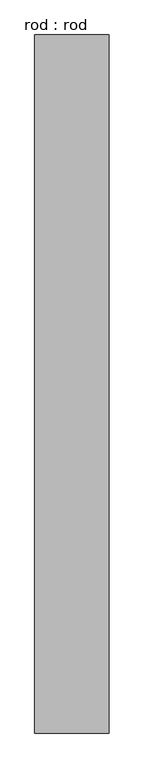
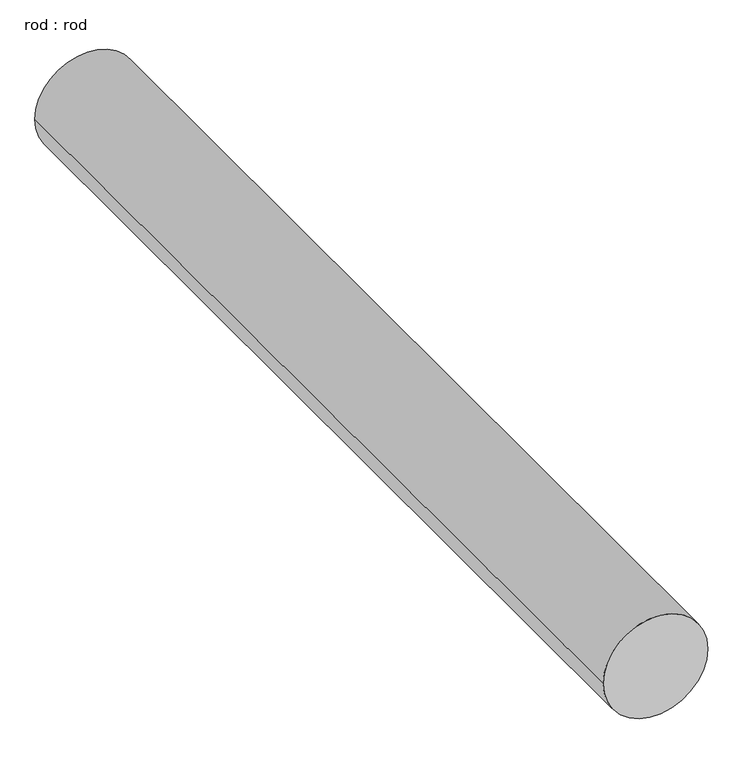
"""IFC4 building model written with IfcOpenShell, lengths in millimetres: proxy geometry, rod : rod."""

from ifc_helpers import new_model, si_unit, point, frame, frame_2d, origin, place, context, project, spatial, circle_curve, trimmed, segment, composite_curve, outline, extrude, source, transform, mapped, element, save


def rod_rod_c9744290(model_context):
    return source(origin(), model_context, "Body", "SweptSolid", [
        extrude(outline(composite_curve([segment(trimmed(circle_curve(frame_2d((0.0108462, 0.0)), 200.0), [point((0.0108462, 200.0))], [point((0.0108462, -200.0))], False, "CARTESIAN"), True, "CONTINUOUS"), segment(trimmed(circle_curve(frame_2d((0.0108462, 0.0)), 200.0), [point((0.0108462, -200.0))], [point((0.0108462, 200.0))], False, "CARTESIAN"), True, "CONTINUOUS")], self_intersect=False)), frame((0.0, 2213.1658337, 0.0), z_axis=(0.0, 1.0, 0.0), x_axis=(0.0, 0.0, 1.0)), (0.0, 0.0, 1.0), 3759.1255632),
    ])


if __name__ == "__main__":
    model = new_model("IFC4")
    model_context = context("Model", 3, world=origin())
    ifc_project = project(units=[si_unit("LENGTHUNIT", "METRE", prefix="MILLI")], contexts=[model_context])
    site = spatial("IfcSite", under=ifc_project)
    building = spatial("IfcBuilding", under=site)
    placement = place(None, origin())
    rod_rod_shape = rod_rod_c9744290(model_context)
    element("IfcBuildingElementProxy", 1, Name="rod : rod", ObjectType="rod : rod", at=placement, inside=building, context=model_context, shape_type="MappedRepresentation", body=[
        mapped(rod_rod_shape, transform((0.0, 0.0, 0.0), x_axis=(1.0, 0.0, 0.0), y_axis=(0.0, 1.0, 0.0), z_axis=(0.0, 0.0, 1.0))),
    ])
    save(model, "model.ifc")

# Revit data of these elements
# Type "rod : rod"
#   Default Elevation = 0
